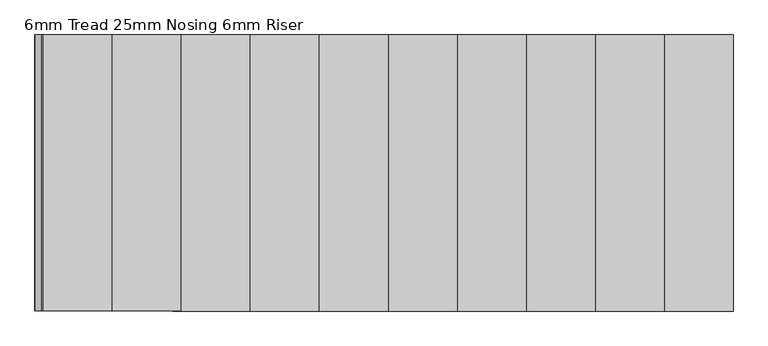
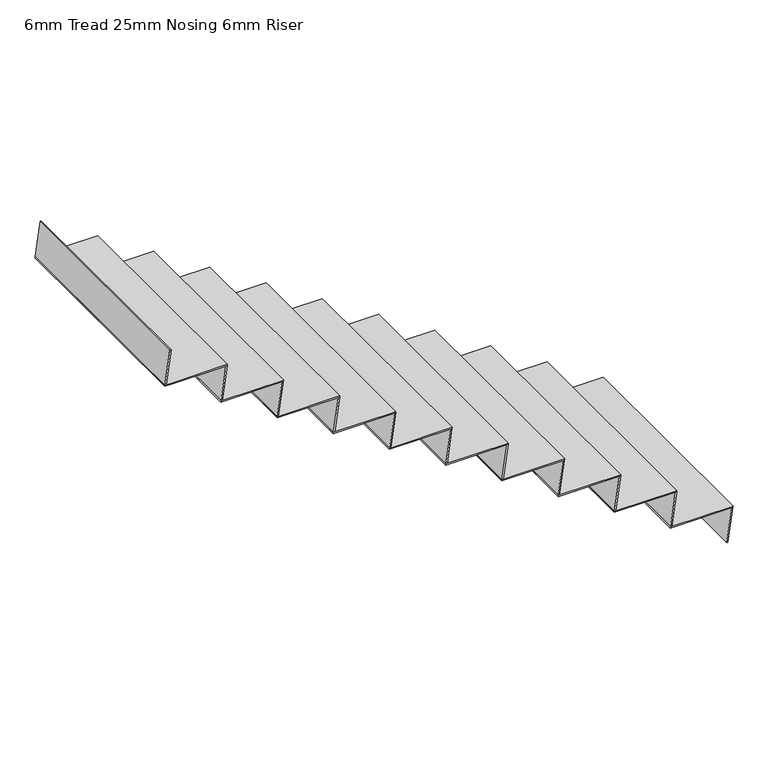
"""IFC4 building model written with IfcOpenShell, lengths in millimetres: stair flight geometry, 6mm Tread 25mm Nosing 6mm Riser."""

from ifc_helpers import new_model, si_unit, origin, place, context, project, spatial, faceted_brep, source, transform, mapped, element, save


def stair_flight_6mm_tread_25mm_nosing_6mm_riser_0fc280bc(model_context):
    return source(origin(), model_context, "Body", "Brep", [
        faceted_brep([(-13906.0590357, 11470.4345331, 177.7777778), (-13906.9027857, 11470.4345331, 171.7777778), (-13906.9027857, 10370.4345331, 171.7777778), (-13906.0590357, 10370.4345331, 177.7777778), (-13600.0, 10370.4345331, 177.7777778), (-13600.0, 11470.4345331, 177.7777778), (-13600.84375, 11470.4345331, 171.7777778), (-13600.84375, 10370.4345331, 171.7777778)], [[[0, 1, 2, 3]], [[3, 4, 5, 0]], [[2, 1, 6, 7]], [[4, 3, 2, 7]], [[0, 5, 6, 1]], [[5, 4, 7, 6]]]),
        faceted_brep([(-13600.84375, 11470.4345331, 171.7777778), (-13625.0, 11470.4345331, 0.0), (-13631.0590357, 11470.4345331, 0.0), (-13606.9027857, 11470.4345331, 171.7777778), (-13600.84375, 10370.4345331, 171.7777778), (-13606.9027857, 10370.4345331, 171.7777778), (-13631.0590357, 10370.4345331, 0.0), (-13625.0, 10370.4345331, 0.0)], [[[0, 1, 2, 3]], [[4, 5, 6, 7]], [[1, 0, 4, 7]], [[2, 1, 7, 6]], [[3, 2, 6, 5]], [[0, 3, 5, 4]]]),
        faceted_brep([(-13875.84375, 11470.4345331, 349.5555556), (-13900.0, 11470.4345331, 177.7777778), (-13906.0590357, 11470.4345331, 177.7777778), (-13881.9027857, 11470.4345331, 349.5555556), (-13875.84375, 10370.4345331, 349.5555556), (-13881.9027857, 10370.4345331, 349.5555556), (-13906.0590357, 10370.4345331, 177.7777778), (-13900.0, 10370.4345331, 177.7777778)], [[[0, 1, 2, 3]], [[4, 5, 6, 7]], [[1, 0, 4, 7]], [[2, 1, 7, 6]], [[3, 2, 6, 5]], [[0, 3, 5, 4]]]),
        faceted_brep([(-14181.0590357, 10370.4345331, 355.5555556), (-13875.0, 10370.4345331, 355.5555556), (-13875.0, 11470.4345331, 355.5555556), (-14181.0590357, 11470.4345331, 355.5555556), (-14181.9027857, 10370.4345331, 349.5555556), (-14181.9027857, 11470.4345331, 349.5555556), (-13875.84375, 11470.4345331, 349.5555556), (-13875.84375, 10370.4345331, 349.5555556)], [[[0, 1, 2, 3]], [[4, 5, 6, 7]], [[1, 0, 4, 7]], [[3, 2, 6, 5]], [[3, 5, 4, 0]], [[2, 1, 7, 6]]]),
        faceted_brep([(-14150.84375, 11470.4345331, 527.3333333), (-14175.0, 11470.4345331, 355.5555556), (-14181.0590357, 11470.4345331, 355.5555556), (-14156.9027857, 11470.4345331, 527.3333333), (-14150.84375, 10370.4345331, 527.3333333), (-14156.9027857, 10370.4345331, 527.3333333), (-14181.0590357, 10370.4345331, 355.5555556), (-14175.0, 10370.4345331, 355.5555556)], [[[0, 1, 2, 3]], [[4, 5, 6, 7]], [[1, 0, 4, 7]], [[2, 1, 7, 6]], [[3, 2, 6, 5]], [[0, 3, 5, 4]]]),
        faceted_brep([(-14456.0590357, 10370.4345331, 533.3333333), (-14150.0, 10370.4345331, 533.3333333), (-14150.0, 11470.4345331, 533.3333333), (-14456.0590357, 11470.4345331, 533.3333333), (-14456.9027857, 10370.4345331, 527.3333333), (-14456.9027857, 11470.4345331, 527.3333333), (-14150.84375, 11470.4345331, 527.3333333), (-14150.84375, 10370.4345331, 527.3333333)], [[[0, 1, 2, 3]], [[4, 5, 6, 7]], [[1, 0, 4, 7]], [[3, 2, 6, 5]], [[3, 5, 4, 0]], [[2, 1, 7, 6]]]),
        faceted_brep([(-14425.84375, 11470.4345331, 705.1111111), (-14450.0, 11470.4345331, 533.3333333), (-14456.0590357, 11470.4345331, 533.3333333), (-14431.9027857, 11470.4345331, 705.1111111), (-14425.84375, 10370.4345331, 705.1111111), (-14431.9027857, 10370.4345331, 705.1111111), (-14456.0590357, 10370.4345331, 533.3333333), (-14450.0, 10370.4345331, 533.3333333)], [[[0, 1, 2, 3]], [[4, 5, 6, 7]], [[1, 0, 4, 7]], [[2, 1, 7, 6]], [[3, 2, 6, 5]], [[0, 3, 5, 4]]]),
        faceted_brep([(-14731.0590357, 10370.4345331, 711.1111111), (-14425.0, 10370.4345331, 711.1111111), (-14425.0, 11470.4345331, 711.1111111), (-14731.0590357, 11470.4345331, 711.1111111), (-14731.9027857, 10370.4345331, 705.1111111), (-14731.9027857, 11470.4345331, 705.1111111), (-14425.84375, 11470.4345331, 705.1111111), (-14425.84375, 10370.4345331, 705.1111111)], [[[0, 1, 2, 3]], [[4, 5, 6, 7]], [[1, 0, 4, 7]], [[3, 2, 6, 5]], [[3, 5, 4, 0]], [[2, 1, 7, 6]]]),
        faceted_brep([(-14700.84375, 11470.4345331, 882.8888889), (-14725.0, 11470.4345331, 711.1111111), (-14731.0590357, 11470.4345331, 711.1111111), (-14706.9027857, 11470.4345331, 882.8888889), (-14700.84375, 10370.4345331, 882.8888889), (-14706.9027857, 10370.4345331, 882.8888889), (-14731.0590357, 10370.4345331, 711.1111111), (-14725.0, 10370.4345331, 711.1111111)], [[[0, 1, 2, 3]], [[4, 5, 6, 7]], [[1, 0, 4, 7]], [[2, 1, 7, 6]], [[3, 2, 6, 5]], [[0, 3, 5, 4]]]),
        faceted_brep([(-15006.0590357, 10370.4345331, 888.8888889), (-14700.0, 10370.4345331, 888.8888889), (-14700.0, 11470.4345331, 888.8888889), (-15006.0590357, 11470.4345331, 888.8888889), (-15006.9027857, 10370.4345331, 882.8888889), (-15006.9027857, 11470.4345331, 882.8888889), (-14700.84375, 11470.4345331, 882.8888889), (-14700.84375, 10370.4345331, 882.8888889)], [[[0, 1, 2, 3]], [[4, 5, 6, 7]], [[1, 0, 4, 7]], [[3, 2, 6, 5]], [[3, 5, 4, 0]], [[2, 1, 7, 6]]]),
        faceted_brep([(-14975.84375, 11470.4345331, 1060.6666667), (-15000.0, 11470.4345331, 888.8888889), (-15006.0590357, 11470.4345331, 888.8888889), (-14981.9027857, 11470.4345331, 1060.6666667), (-14975.84375, 10370.4345331, 1060.6666667), (-14981.9027857, 10370.4345331, 1060.6666667), (-15006.0590357, 10370.4345331, 888.8888889), (-15000.0, 10370.4345331, 888.8888889)], [[[0, 1, 2, 3]], [[4, 5, 6, 7]], [[1, 0, 4, 7]], [[2, 1, 7, 6]], [[3, 2, 6, 5]], [[0, 3, 5, 4]]]),
        faceted_brep([(-15281.0590357, 10370.4345331, 1066.6666667), (-14975.0, 10370.4345331, 1066.6666667), (-14975.0, 11470.4345331, 1066.6666667), (-15281.0590357, 11470.4345331, 1066.6666667), (-15281.9027857, 10370.4345331, 1060.6666667), (-15281.9027857, 11470.4345331, 1060.6666667), (-14975.84375, 11470.4345331, 1060.6666667), (-14975.84375, 10370.4345331, 1060.6666667)], [[[0, 1, 2, 3]], [[4, 5, 6, 7]], [[1, 0, 4, 7]], [[3, 2, 6, 5]], [[3, 5, 4, 0]], [[2, 1, 7, 6]]]),
        faceted_brep([(-15250.84375, 11470.4345331, 1238.4444444), (-15275.0, 11470.4345331, 1066.6666667), (-15281.0590357, 11470.4345331, 1066.6666667), (-15256.9027857, 11470.4345331, 1238.4444444), (-15250.84375, 10370.4345331, 1238.4444444), (-15256.9027857, 10370.4345331, 1238.4444444), (-15281.0590357, 10370.4345331, 1066.6666667), (-15275.0, 10370.4345331, 1066.6666667)], [[[0, 1, 2, 3]], [[4, 5, 6, 7]], [[1, 0, 4, 7]], [[2, 1, 7, 6]], [[3, 2, 6, 5]], [[0, 3, 5, 4]]]),
        faceted_brep([(-15556.0590357, 10370.4345331, 1244.4444444), (-15250.0, 10370.4345331, 1244.4444444), (-15250.0, 11470.4345331, 1244.4444444), (-15556.0590357, 11470.4345331, 1244.4444444), (-15556.9027857, 10370.4345331, 1238.4444444), (-15556.9027857, 11470.4345331, 1238.4444444), (-15250.84375, 11470.4345331, 1238.4444444), (-15250.84375, 10370.4345331, 1238.4444444)], [[[0, 1, 2, 3]], [[4, 5, 6, 7]], [[1, 0, 4, 7]], [[3, 2, 6, 5]], [[3, 5, 4, 0]], [[2, 1, 7, 6]]]),
        faceted_brep([(-15525.84375, 11470.4345331, 1416.2222222), (-15550.0, 11470.4345331, 1244.4444444), (-15556.0590357, 11470.4345331, 1244.4444444), (-15531.9027857, 11470.4345331, 1416.2222222), (-15525.84375, 10370.4345331, 1416.2222222), (-15531.9027857, 10370.4345331, 1416.2222222), (-15556.0590357, 10370.4345331, 1244.4444444), (-15550.0, 10370.4345331, 1244.4444444)], [[[0, 1, 2, 3]], [[4, 5, 6, 7]], [[1, 0, 4, 7]], [[2, 1, 7, 6]], [[3, 2, 6, 5]], [[0, 3, 5, 4]]]),
        faceted_brep([(-15831.0590357, 10370.4345331, 1422.2222222), (-15525.0, 10370.4345331, 1422.2222222), (-15525.0, 11470.4345331, 1422.2222222), (-15831.0590357, 11470.4345331, 1422.2222222), (-15831.9027857, 10370.4345331, 1416.2222222), (-15831.9027857, 11470.4345331, 1416.2222222), (-15525.84375, 11470.4345331, 1416.2222222), (-15525.84375, 10370.4345331, 1416.2222222)], [[[0, 1, 2, 3]], [[4, 5, 6, 7]], [[1, 0, 4, 7]], [[3, 2, 6, 5]], [[3, 5, 4, 0]], [[2, 1, 7, 6]]]),
        faceted_brep([(-15800.84375, 11470.4345331, 1594.0), (-15825.0, 11470.4345331, 1422.2222222), (-15831.0590357, 11470.4345331, 1422.2222222), (-15806.9027857, 11470.4345331, 1594.0), (-15800.84375, 10370.4345331, 1594.0), (-15806.9027857, 10370.4345331, 1594.0), (-15831.0590357, 10370.4345331, 1422.2222222), (-15825.0, 10370.4345331, 1422.2222222)], [[[0, 1, 2, 3]], [[4, 5, 6, 7]], [[1, 0, 4, 7]], [[2, 1, 7, 6]], [[3, 2, 6, 5]], [[0, 3, 5, 4]]]),
        faceted_brep([(-16106.0590357, 10370.4345331, 1600.0), (-15800.0, 10370.4345331, 1600.0), (-15800.0, 11470.4345331, 1600.0), (-16106.0590357, 11470.4345331, 1600.0), (-16106.9027857, 10370.4345331, 1594.0), (-16106.9027857, 11470.4345331, 1594.0), (-15800.84375, 11470.4345331, 1594.0), (-15800.84375, 10370.4345331, 1594.0)], [[[0, 1, 2, 3]], [[4, 5, 6, 7]], [[1, 0, 4, 7]], [[3, 2, 6, 5]], [[3, 5, 4, 0]], [[2, 1, 7, 6]]]),
        faceted_brep([(-16350.84375, 11470.4345331, 1949.5555556), (-16375.0, 11470.4345331, 1777.7777778), (-16381.0590357, 11470.4345331, 1777.7777778), (-16356.9027857, 11470.4345331, 1949.5555556), (-16350.84375, 10370.4345331, 1949.5555556), (-16356.9027857, 10370.4345331, 1949.5555556), (-16381.0590357, 10370.4345331, 1777.7777778), (-16375.0, 10370.4345331, 1777.7777778)], [[[0, 1, 2, 3]], [[4, 5, 6, 7]], [[1, 0, 4, 7]], [[2, 1, 7, 6]], [[3, 2, 6, 5]], [[0, 3, 5, 4]]]),
        faceted_brep([(-16075.84375, 11470.4345331, 1771.7777778), (-16100.0, 11470.4345331, 1600.0), (-16106.0590357, 11470.4345331, 1600.0), (-16081.9027857, 11470.4345331, 1771.7777778), (-16075.84375, 10370.4345331, 1771.7777778), (-16081.9027857, 10370.4345331, 1771.7777778), (-16106.0590357, 10370.4345331, 1600.0), (-16100.0, 10370.4345331, 1600.0)], [[[0, 1, 2, 3]], [[4, 5, 6, 7]], [[1, 0, 4, 7]], [[2, 1, 7, 6]], [[3, 2, 6, 5]], [[0, 3, 5, 4]]]),
        faceted_brep([(-16381.0590357, 10370.4345331, 1777.7777778), (-16350.0, 10370.4345331, 1777.7777778), (-16075.0, 10370.4345331, 1777.7777778), (-16075.0, 11470.4345331, 1777.7777778), (-16381.0590357, 11470.4345331, 1777.7777778), (-16381.9027857, 10370.4345331, 1771.7777778), (-16381.9027857, 11470.4345331, 1771.7777778), (-16075.84375, 11470.4345331, 1771.7777778), (-16075.84375, 10370.4345331, 1771.7777778), (-16350.0, 10370.4345331, 1771.7777778)], [[[0, 1, 2, 3, 4]], [[5, 6, 7, 8, 9]], [[1, 0, 5, 9]], [[2, 1, 9, 8]], [[4, 3, 7, 6]], [[4, 6, 5, 0]], [[3, 2, 8, 7]]]),
    ])


if __name__ == "__main__":
    model = new_model("IFC4")
    model_context = context("Model", 3, world=origin())
    ifc_project = project(units=[si_unit("LENGTHUNIT", "METRE", prefix="MILLI")], contexts=[model_context])
    site = spatial("IfcSite", under=ifc_project)
    building = spatial("IfcBuilding", under=site)
    placement = place(None, origin())
    stair_flight_6mm_tread_25mm_nosing_6mm_riser_shape = stair_flight_6mm_tread_25mm_nosing_6mm_riser_0fc280bc(model_context)
    element("IfcStairFlight", 1, ObjectType="6mm Tread 25mm Nosing 6mm Riser", at=placement, inside=building, context=model_context, shape_type="MappedRepresentation", body=[
        mapped(stair_flight_6mm_tread_25mm_nosing_6mm_riser_shape, transform((0.0, 0.0, 0.0), x_axis=(1.0, 0.0, 0.0), y_axis=(0.0, 1.0, 0.0), z_axis=(0.0, 0.0, 1.0))),
    ])
    save(model, "model.ifc")

# Revit data of these elements
# Element 1 (IfcStairFlight, "6mm Tread 25mm Nosing 6mm Riser")
#   Materials on its faces: "Steel, Paint Finish, Dark Gray"
# Materials
#   "Steel, Paint Finish, Dark Gray": class "Metal", colour RGB 89 89 89, transparency 0, Description = "Steel, paint finish, dark gray, glossy", Cost = 0
